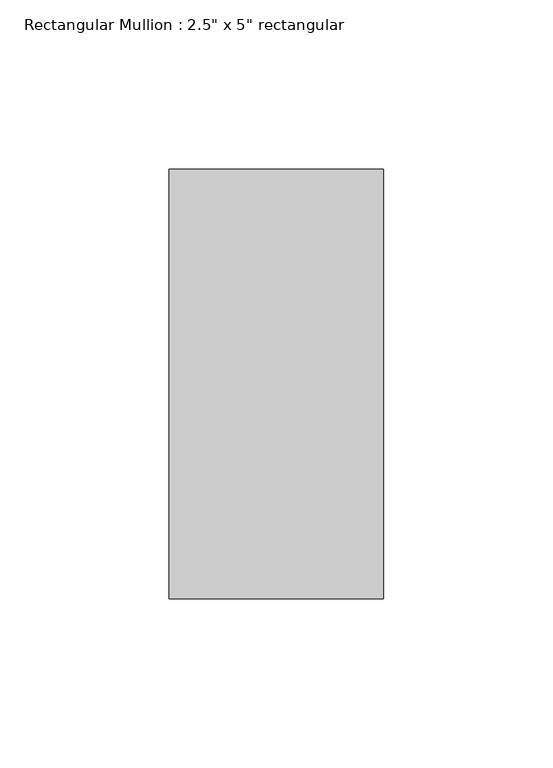
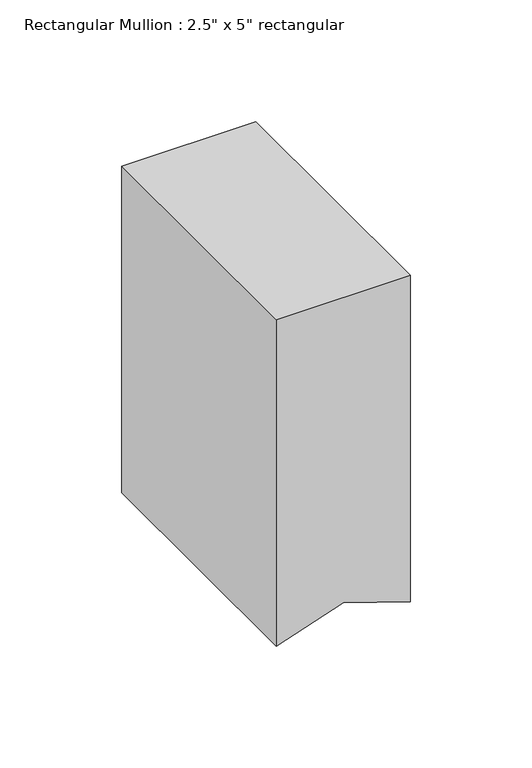
"""IFC4 building model written with IfcOpenShell, lengths in millimetres: member geometry."""

import ifcopenshell
import ifcopenshell.guid

model = None  # the IFC model being written
_history = None  # IfcOwnerHistory: only IFC2X3 demands one
_inside = {}  # id of a spatial element -> (the spatial element, [elements in it])
_under = {}  # id of a project, library or spatial element -> (it, [spatial elements below it])
_declared = {}  # id of a project -> (the project, [libraries it declares])
_typed = {}  # id of a type object -> (the type object, [elements of that type])
_made_of = {}  # id of a material, layer set ... -> (it, [elements and type objects made of it])


def new_model(schema):
    """Start an empty IFC model of exactly this schema.

    Asked for "IFC4X3", IfcOpenShell would pick the latest addendum, in which some entities
    have other attributes; the version numbers below select the first issue.
    IFC2X3 requires an IfcOwnerHistory on every rooted entity: one is made here for all.
    """
    global model, _history
    if schema == "IFC4X3":
        model = ifcopenshell.file(schema_version=(4, 3, 0, 0))
    else:
        model = ifcopenshell.file(schema=schema)
    _inside.clear()
    _under.clear()
    _declared.clear()
    _typed.clear()
    _made_of.clear()
    _history = None
    if model.schema == "IFC2X3":
        org = make("IfcOrganization", Name="unknown")
        user = make(
            "IfcPersonAndOrganization",
            ThePerson=make("IfcPerson", FamilyName="unknown"),
            TheOrganization=org,
        )
        app = make(
            "IfcApplication",
            ApplicationDeveloper=org,
            Version="unknown",
            ApplicationFullName="unknown",
            ApplicationIdentifier="unknown",
        )
        _history = make(
            "IfcOwnerHistory",
            OwningUser=user,
            OwningApplication=app,
            ChangeAction="ADDED",
            CreationDate=0,
        )
    return model


def make(cls, **values):
    """One entity of the class cls with the attributes given. An attribute that is None is left unset."""
    return model.create_entity(
        cls, **{name: value for name, value in values.items() if value is not None}
    )


def rooted(cls, **values):
    """An entity with a GlobalId (a new one), such as an element, a storey or a relation."""
    return make(cls, GlobalId=ifcopenshell.guid.new(), OwnerHistory=_history, **values)


def si_unit(unit_type, name, prefix=None):
    """IfcSIUnit, for example si_unit("LENGTHUNIT", "METRE", prefix="MILLI")."""
    return make("IfcSIUnit", UnitType=unit_type, Prefix=prefix, Name=name)


def assignment(units):
    """IfcUnitAssignment: the units of a project."""
    return None if units is None else make("IfcUnitAssignment", Units=units)


def point(xyz):
    """IfcCartesianPoint."""
    return None if xyz is None else make("IfcCartesianPoint", Coordinates=xyz)


def direction(xyz):
    """IfcDirection."""
    return None if xyz is None else make("IfcDirection", DirectionRatios=xyz)


def frame(location, z_axis=None, x_axis=None):
    """IfcAxis2Placement3D, a coordinate frame: its origin and axes. An axis left out is left unset."""
    return make(
        "IfcAxis2Placement3D",
        Location=point(location),
        Axis=direction(z_axis),
        RefDirection=direction(x_axis),
    )


def origin():
    """The frame at (0, 0, 0) with its axes left unset."""
    return frame((0.0, 0.0, 0.0))


def place(relative_to, where):
    """IfcLocalPlacement: puts the frame where relative to a parent placement (None: the world)."""
    return make(
        "IfcLocalPlacement", PlacementRelTo=relative_to, RelativePlacement=where
    )


def context(
    kind, dimensions, precision=None, world=None, true_north=None, identifier=None
):
    """IfcGeometricRepresentationContext, for example the 3D "Model" context."""
    return make(
        "IfcGeometricRepresentationContext",
        ContextIdentifier=identifier,
        ContextType=kind,
        CoordinateSpaceDimension=dimensions,
        Precision=precision,
        WorldCoordinateSystem=world,
        TrueNorth=true_north,
    )


def project(units=None, contexts=None):
    """IfcProject with its units and contexts."""
    return rooted(
        "IfcProject",
        Name="project",
        RepresentationContexts=contexts,
        UnitsInContext=assignment(units),
    )


def spatial(cls, under=None, at=None, **own):
    """A site, building, storey or space (cls), placed at a placement, below another one or the project."""
    s = rooted(cls, ObjectPlacement=at, **own)
    if under is not None:
        _under.setdefault(under.id(), (under, []))[1].append(s)
    return s


def polyline(points):
    """IfcPolyline through the points."""
    return make("IfcPolyline", Points=[point(p) for p in points])


def outline(outer, holes=None, kind="AREA"):
    """IfcArbitraryClosedProfileDef: a profile drawn as a closed curve; with holes, ...WithVoids."""
    if holes is None:
        return make("IfcArbitraryClosedProfileDef", ProfileType=kind, OuterCurve=outer)
    return make(
        "IfcArbitraryProfileDefWithVoids",
        ProfileType=kind,
        OuterCurve=outer,
        InnerCurves=holes,
    )


def extrude(swept, where, along, depth):
    """IfcExtrudedAreaSolid: the profile swept, set in the frame where, extruded along a direction by depth."""
    return make(
        "IfcExtrudedAreaSolid",
        SweptArea=swept,
        Position=where,
        ExtrudedDirection=direction(along),
        Depth=depth,
    )


def shape(context_of_items, identifier, shape_type, items):
    """IfcShapeRepresentation: the items that make up one representation, for example the "Body"."""
    return make(
        "IfcShapeRepresentation",
        ContextOfItems=context_of_items,
        RepresentationIdentifier=identifier,
        RepresentationType=shape_type,
        Items=items,
    )


def source(mapping_origin, context_of_items, identifier, shape_type, items):
    """IfcRepresentationMap: a shape defined once, which mapped items show again and again."""
    return make(
        "IfcRepresentationMap",
        MappingOrigin=mapping_origin,
        MappedRepresentation=shape(context_of_items, identifier, shape_type, items),
    )


def transform(
    local_origin,
    x_axis=None,
    y_axis=None,
    z_axis=None,
    scale=None,
    scale2=None,
    scale3=None,
    uniform=True,
):
    """IfcCartesianTransformationOperator3D, or its non-uniform kind. x_axis, y_axis, z_axis: its Axis1, 2, 3."""
    if uniform:
        return make(
            "IfcCartesianTransformationOperator3D",
            Axis1=direction(x_axis),
            Axis2=direction(y_axis),
            LocalOrigin=point(local_origin),
            Scale=scale,
            Axis3=direction(z_axis),
        )
    return make(
        "IfcCartesianTransformationOperator3DnonUniform",
        Axis1=direction(x_axis),
        Axis2=direction(y_axis),
        LocalOrigin=point(local_origin),
        Scale=scale,
        Axis3=direction(z_axis),
        Scale2=scale2,
        Scale3=scale3,
    )


def mapped(mapping_source, mapping_target):
    """IfcMappedItem: shows the shape of a source again, moved by a transform."""
    return make(
        "IfcMappedItem", MappingSource=mapping_source, MappingTarget=mapping_target
    )


def made_of(thing, what):
    """Note that an element or type object is made of a material, layer set ...; save() writes the relation."""
    if what is not None:
        _made_of.setdefault(what.id(), (what, []))[1].append(thing)
    return thing


def element(
    cls,
    number,
    at=None,
    inside=None,
    cuts=None,
    type_object=None,
    material=None,
    context=None,
    identifier="Body",
    shape_type=None,
    held_by="IfcProductDefinitionShape",
    body=None,
    shapes=None,
    **own,
):
    """One element of the class cls, such as IfcWall. Its Tag is "e" and its number.

    at: its placement. inside: the storey or other place that contains it. cuts: it is an
    opening in that element (IfcRelVoidsElement). A single representation is given by context,
    identifier, shape_type and body (its items); several are given by shapes. held_by: the class
    of the entity that holds the representations. save() writes the other relations.
    """
    e = rooted(cls, Tag="e%d" % number, ObjectPlacement=at, **own)
    if body is not None:
        shapes = [shape(context, identifier, shape_type, body)]
    if shapes is not None:
        e.Representation = make(held_by, Representations=shapes)
    if inside is not None:
        _inside.setdefault(inside.id(), (inside, []))[1].append(e)
    if cuts is not None:
        rooted(
            "IfcRelVoidsElement", RelatingBuildingElement=cuts, RelatedOpeningElement=e
        )
    if type_object is not None:
        _typed.setdefault(type_object.id(), (type_object, []))[1].append(e)
    return made_of(e, material)


def aggregate(whole, parts):
    """IfcRelAggregates: a whole, such as a stair, and the parts it consists of."""
    return rooted("IfcRelAggregates", RelatingObject=whole, RelatedObjects=parts)


def save(model, path):
    """Write the relations noted so far, then the file.

    IfcRelAggregates (storeys below a building ...), IfcRelContainedInSpatialStructure (elements
    in a storey), IfcRelDefinesByType, IfcRelAssociatesMaterial and IfcRelDeclares: one each for
    every whole, place, type object, material and project.
    """
    for whole, parts in _under.values():
        aggregate(whole, parts)
    for where, things in _inside.values():
        rooted(
            "IfcRelContainedInSpatialStructure",
            RelatedElements=things,
            RelatingStructure=where,
        )
    for kind, things in _typed.values():
        rooted("IfcRelDefinesByType", RelatedObjects=things, RelatingType=kind)
    for what, things in _made_of.values():
        rooted("IfcRelAssociatesMaterial", RelatedObjects=things, RelatingMaterial=what)
    for by, libraries in _declared.values():
        rooted("IfcRelDeclares", RelatingContext=by, RelatedDefinitions=libraries)
    model.write(path)


def member_f4359540(model_context):
    return source(origin(), model_context, "Body", "SweptSolid", [
        extrude(outline(polyline([(0.0, 31.75), (0.0, -31.75), (-163.7817895, -31.75), (-153.1984562, 0.0), (-163.7817895, 31.75), (0.0, 31.75)])), frame((0.0, -63.5, 0.0), z_axis=(0.0, 1.0, 0.0), x_axis=(0.0, 0.0, 1.0)), (0.0, 0.0, 1.0), 127.0),
    ])


if __name__ == "__main__":
    model = new_model("IFC4")
    model_context = context("Model", 3, world=origin())
    ifc_project = project(units=[si_unit("LENGTHUNIT", "METRE", prefix="MILLI")], contexts=[model_context])
    site = spatial("IfcSite", under=ifc_project)
    building = spatial("IfcBuilding", under=site)
    placement = place(None, origin())
    member_shape = member_f4359540(model_context)
    element("IfcMember", 1, ObjectType="Rectangular Mullion : 2.5\" x 5\" rectangular", at=placement, inside=building, context=model_context, shape_type="MappedRepresentation", body=[
        mapped(member_shape, transform((0.0, 0.0, 0.0), x_axis=(1.0, 0.0, 0.0), y_axis=(0.0, 1.0, 0.0), z_axis=(0.0, 0.0, 1.0))),
    ])
    save(model, "model.ifc")

# Revit data of these elements
# Type "Rectangular Mullion : 2.5\" x 5\" rectangular"
#   built-in parameter 1007304 = 0.416667 (stored number, unit not read)
#   built-in parameter 1007301 = 0.104167 (stored number, unit not read)
#   built-in parameter 1007300 = 0.104167 (stored number, unit not read)
# Element 1 (IfcMember, "Rectangular Mullion : 2.5\" x 5\" rectangular")
#   Materials on its faces: "Metal - Aluminum"
# Materials
#   "Metal - Aluminum": class "Metal", colour RGB 140 140 140, transparency 0
